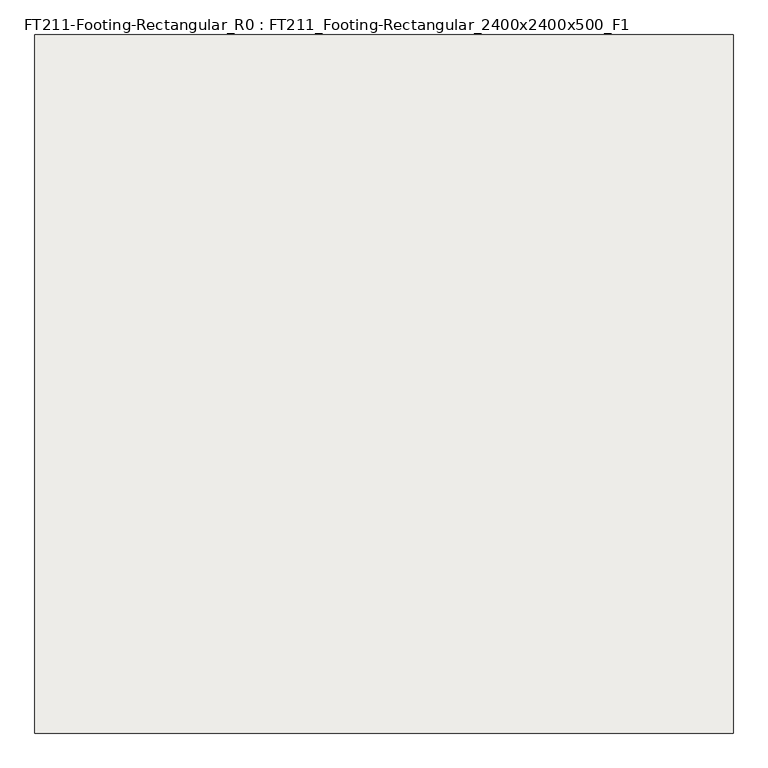
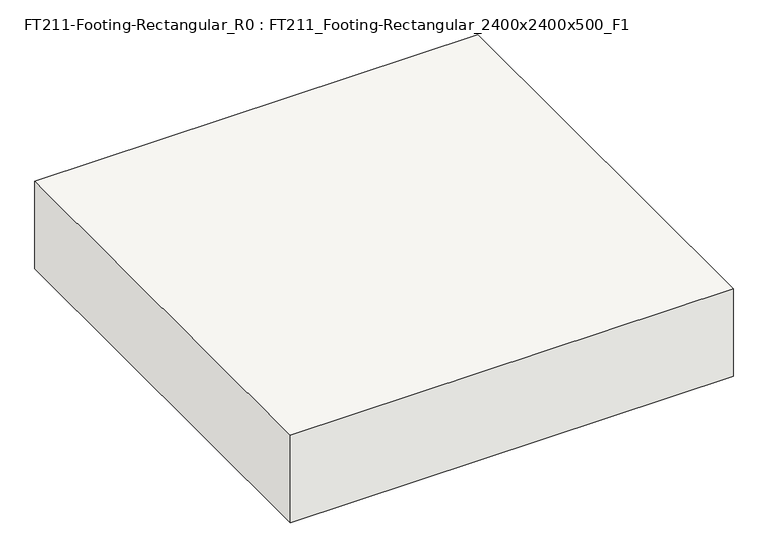
"""IFC4 building model written with IfcOpenShell, lengths in millimetres: slab geometry, FT211-Footing-Rectangular_R0 : FT211_Footing-Rectangular_2400x2400x500_F1."""

from ifc_helpers import new_model, si_unit, frame, origin, place, context, project, spatial, polyline, outline, extrude, source, transform, mapped, element, save


def ft211_footing_rectangular_r0_ft211_footing_rectangular_5fe39465(model_context):
    return source(origin(), model_context, "Body", "SweptSolid", [
        extrude(outline(polyline([(1200.0, 1200.0), (1200.0, -1200.0), (-1200.0, -1200.0), (-1200.0, 1200.0), (1200.0, 1200.0)])), frame((0.0, 0.0, -500.0), z_axis=(0.0, 0.0, 1.0), x_axis=(1.0, 0.0, 0.0)), (0.0, 0.0, 1.0), 500.0),
    ])


if __name__ == "__main__":
    model = new_model("IFC4")
    model_context = context("Model", 3, world=origin())
    ifc_project = project(units=[si_unit("LENGTHUNIT", "METRE", prefix="MILLI")], contexts=[model_context])
    site = spatial("IfcSite", under=ifc_project)
    building = spatial("IfcBuilding", under=site)
    placement = place(None, origin())
    ft211_footing_rectangular_r0_ft211_footing_rectangular_shape = ft211_footing_rectangular_r0_ft211_footing_rectangular_5fe39465(model_context)
    element("IfcSlab", 1, ObjectType="FT211-Footing-Rectangular_R0 : FT211_Footing-Rectangular_2400x2400x500_F1", at=placement, inside=building, context=model_context, shape_type="MappedRepresentation", body=[
        mapped(ft211_footing_rectangular_r0_ft211_footing_rectangular_shape, transform((0.0, 0.0, 0.0), x_axis=(1.0, 0.0, 0.0), y_axis=(0.0, 1.0, 0.0), z_axis=(0.0, 0.0, 1.0))),
    ])
    save(model, "model.ifc")

# Revit data of these elements
# Type "FT211-Footing-Rectangular_R0 : FT211_Footing-Rectangular_2400x2400x500_F1"
#   Top bar = "D25@300"
#   Description = "UG Shallow Foundation"
#   Bottom bar = "D20@300"
#   Width = 2400 mm
#   Length = 2400 mm
#   Foundation Thickness = 500 mm
#   Structural Material [instance default] = A03AC032-00007_Structural Concrete_Type1_25MPa-30Mpa
#   Assembly Code = ""
# Element 1 (IfcSlab, "FT211-Footing-Rectangular_R0 : FT211_Footing-Rectangular_2400x2400x500_F1")
#   Materials on its faces: "A03AC032-00007_Structural Concrete_Type1_25MPa-30Mpa"
# Materials
#   "A03AC032-00007_Structural Concrete_Type1_25MPa-30Mpa": class "Concrete", colour RGB 176 176 176, transparency 0, Keynote = "09910.A1", Description = "Reinf. Conc.", W00) Work Master Code = "A03AC032-00007", W01) Work Master_Lv1 = "Concrete Work", W02) Work Master_Lv2 = "Substructure Work", W03) Work Master_Spec.1 = "Structural Concrete", W04) Work Master_Spec.2 = "Cement Type-1", W05) Work Master_Spec.3 = "25MPa < F'c (Cylinder Strength) ≤ 30MPa", Cost = 0
